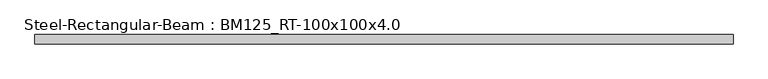
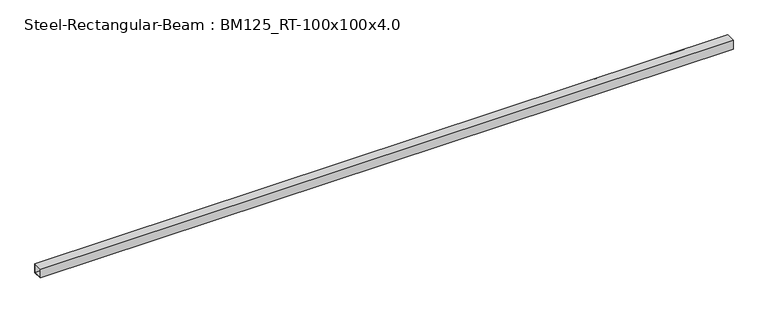
"""IFC4 building model written with IfcOpenShell, lengths in millimetres: beam geometry, Steel-Rectangular-Beam : BM125_RT-100x100x4.0."""

from ifc_helpers import new_model, si_unit, frame, origin, place, context, project, spatial, polyline, outline, extrude, source, transform, mapped, element, save


def steel_rectangular_beam_bm125_rt_100x100x4_0_60a5dd41(model_context):
    return source(origin(), model_context, "Body", "SweptSolid", [
        extrude(outline(polyline([(-50.0, 50.0), (50.0, 50.0), (50.0, -50.0), (-50.0, -50.0), (-50.0, 50.0)]), holes=[polyline([(46.0, -46.0), (46.0, 46.0), (-46.0, 46.0), (-46.0, -46.0), (46.0, -46.0)])]), frame((-3725.0, 0.0, 0.0), z_axis=(1.0, 0.0, 0.0), x_axis=(0.0, 1.0, 0.0)), (0.0, 0.0, 1.0), 7450.0),
        extrude(outline(polyline([(-50.0, 50.0), (50.0, 50.0), (50.0, -50.0), (-50.0, -50.0), (-50.0, 50.0)]), holes=[polyline([(46.0, -46.0), (46.0, 46.0), (-46.0, 46.0), (-46.0, -46.0), (46.0, -46.0)])]), frame((-3725.0, 0.0, 0.0), z_axis=(1.0, 0.0, 0.0), x_axis=(0.0, 1.0, 0.0)), (0.0, 0.0, 1.0), 7450.0),
        extrude(outline(polyline([(-50.0, 50.0), (50.0, 50.0), (50.0, -50.0), (-50.0, -50.0), (-50.0, 50.0)]), holes=[polyline([(46.0, -46.0), (46.0, 46.0), (-46.0, 46.0), (-46.0, -46.0), (46.0, -46.0)])]), frame((-3725.0, 0.0, 0.0), z_axis=(1.0, 0.0, 0.0), x_axis=(0.0, 1.0, 0.0)), (0.0, 0.0, 1.0), 7450.0),
        extrude(outline(polyline([(-50.0, 50.0), (50.0, 50.0), (50.0, -50.0), (-50.0, -50.0), (-50.0, 50.0)]), holes=[polyline([(46.0, -46.0), (46.0, 46.0), (-46.0, 46.0), (-46.0, -46.0), (46.0, -46.0)])]), frame((-3725.0, 0.0, 0.0), z_axis=(1.0, 0.0, 0.0), x_axis=(0.0, 1.0, 0.0)), (0.0, 0.0, 1.0), 7450.0),
    ])


if __name__ == "__main__":
    model = new_model("IFC4")
    model_context = context("Model", 3, world=origin())
    ifc_project = project(units=[si_unit("LENGTHUNIT", "METRE", prefix="MILLI")], contexts=[model_context])
    site = spatial("IfcSite", under=ifc_project)
    building = spatial("IfcBuilding", under=site)
    placement = place(None, origin())
    steel_rectangular_beam_bm125_rt_100x100x4_0_shape = steel_rectangular_beam_bm125_rt_100x100x4_0_60a5dd41(model_context)
    element("IfcBeam", 1, ObjectType="Steel-Rectangular-Beam : BM125_RT-100x100x4.0", at=placement, inside=building, context=model_context, shape_type="MappedRepresentation", body=[
        mapped(steel_rectangular_beam_bm125_rt_100x100x4_0_shape, transform((0.0, 0.0, 0.0), x_axis=(1.0, 0.0, 0.0), y_axis=(0.0, 1.0, 0.0), z_axis=(0.0, 0.0, 1.0))),
    ])
    save(model, "model.ifc")

# Revit data of these elements
# Type "Steel-Rectangular-Beam : BM125_RT-100x100x4.0"
#   t = 4 mm
#   Mass per Unit Length = 11.70 kg/m
#   Surface Area = 0.386 m²/m
#   Sectional Area = 14.95 cm²
#   Length [instance default] = 3000 mm
#   H = 100 mm
#   B = 100 mm
#   hec_material4 [instance default] = none
#   hec_material3 [instance default] = none
#   hec_material2 [instance default] = none
#   hec_material1 [instance default] = none
#   Structural Material [instance default] = none
# Element 1 (IfcBeam, "Steel-Rectangular-Beam : BM125_RT-100x100x4.0")
#   hec_material2 = S01AA010-00001_Main Steel Structure Fabrication Work_Shelter/Building_Steel Painting/Coating_for Non-Fireproofed Steel Surface, Surface Preparation, Primer, Second & Final Coat
#   hec_material1 = S03AA007-00001_Main Steel Structure Erection Work_Girth & Purlin
#   Structural Material = S01AA007-00001_Main Steel Structure Fabrication Work_Shelter/Building_Girth & Purlin
#   Materials on its faces: "S01AA010-00001_Main Steel Structure Fabrication Work_Shelter/Building_Steel Painting/Coating_for Non-Fireproofed Steel Surface, Surface Preparation, Primer, Second & Final Coat"
# Materials
#   "S01AA010-00001_Main Steel Structure Fabrication Work_Shelter/Building_Steel Painting/Coating_for Non-Fireproofed Steel Surface, Surface Preparation, Primer, Second & Final Coat": class "Metal", colour RGB 120 120 120, transparency 0, Description = "Paint finished steel", W00) Work Master Code = "S01AA010-00001", W01) Work Master_Lv1 = "Main Steel Structure Fabrication Work", W02) Work Master_Lv2 = "Shelter/Building", W03) Work Master_Spec.1 = "Steel Painting/Coating", W04) Work Master_Spec.2 = "for Non-Fireproofed Steel Surface, Surface Preparation, Primer, Second & Final Coat", Cost = 0
#   "S03AA007-00001_Main Steel Structure Erection Work_Girth & Purlin": class "Metal", colour RGB 120 120 120, transparency 0, Comments = "(30KG/M>Weight)", Description = "Structural steel 50ksi", W00) Work Master Code = "S03AA007-00001", W01) Work Master_Lv1 = "Main Steel Structure Erection Work", W02) Work Master_Lv2 = "Shelter/Building", W03) Work Master_Spec.1 = "Girth & Purlin", Cost = 0
#   "S01AA007-00001_Main Steel Structure Fabrication Work_Shelter/Building_Girth & Purlin": class "Metal", colour RGB 120 120 120, transparency 0, Comments = "(30KG/M>Weight)", Description = "Structural steel 50ksi", W00) Work Master Code = "S01AA007-00001", W01) Work Master_Lv1 = "Main Steel Structure Fabrication Work", W02) Work Master_Lv2 = "Shelter/Building", W03) Work Master_Spec.1 = "Girth & Purlin", Cost = 0
